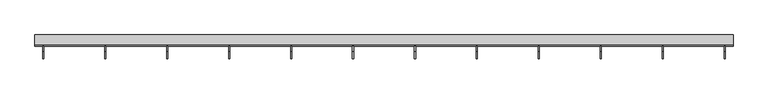
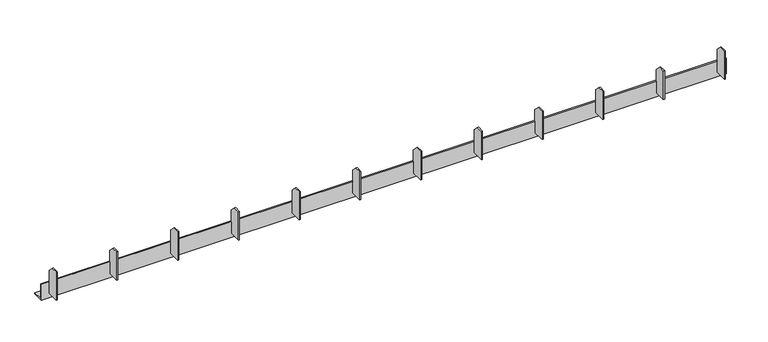
"""IFC4 building model written with IfcOpenShell, lengths in millimetres: beam geometry, NLRS_31_SF_LIB_latei geveldrager staal-AV-CWV-MMBS-SRP_gen_rsf : geveldrager_gen."""

import ifcopenshell
import ifcopenshell.guid

model = None  # the IFC model being written
_history = None  # IfcOwnerHistory: only IFC2X3 demands one
_inside = {}  # id of a spatial element -> (the spatial element, [elements in it])
_under = {}  # id of a project, library or spatial element -> (it, [spatial elements below it])
_declared = {}  # id of a project -> (the project, [libraries it declares])
_typed = {}  # id of a type object -> (the type object, [elements of that type])
_made_of = {}  # id of a material, layer set ... -> (it, [elements and type objects made of it])


def new_model(schema):
    """Start an empty IFC model of exactly this schema.

    Asked for "IFC4X3", IfcOpenShell would pick the latest addendum, in which some entities
    have other attributes; the version numbers below select the first issue.
    IFC2X3 requires an IfcOwnerHistory on every rooted entity: one is made here for all.
    """
    global model, _history
    if schema == "IFC4X3":
        model = ifcopenshell.file(schema_version=(4, 3, 0, 0))
    else:
        model = ifcopenshell.file(schema=schema)
    _inside.clear()
    _under.clear()
    _declared.clear()
    _typed.clear()
    _made_of.clear()
    _history = None
    if model.schema == "IFC2X3":
        org = make("IfcOrganization", Name="unknown")
        user = make(
            "IfcPersonAndOrganization",
            ThePerson=make("IfcPerson", FamilyName="unknown"),
            TheOrganization=org,
        )
        app = make(
            "IfcApplication",
            ApplicationDeveloper=org,
            Version="unknown",
            ApplicationFullName="unknown",
            ApplicationIdentifier="unknown",
        )
        _history = make(
            "IfcOwnerHistory",
            OwningUser=user,
            OwningApplication=app,
            ChangeAction="ADDED",
            CreationDate=0,
        )
    return model


def make(cls, **values):
    """One entity of the class cls with the attributes given. An attribute that is None is left unset."""
    return model.create_entity(
        cls, **{name: value for name, value in values.items() if value is not None}
    )


def rooted(cls, **values):
    """An entity with a GlobalId (a new one), such as an element, a storey or a relation."""
    return make(cls, GlobalId=ifcopenshell.guid.new(), OwnerHistory=_history, **values)


def si_unit(unit_type, name, prefix=None):
    """IfcSIUnit, for example si_unit("LENGTHUNIT", "METRE", prefix="MILLI")."""
    return make("IfcSIUnit", UnitType=unit_type, Prefix=prefix, Name=name)


def assignment(units):
    """IfcUnitAssignment: the units of a project."""
    return None if units is None else make("IfcUnitAssignment", Units=units)


def point(xyz):
    """IfcCartesianPoint."""
    return None if xyz is None else make("IfcCartesianPoint", Coordinates=xyz)


def direction(xyz):
    """IfcDirection."""
    return None if xyz is None else make("IfcDirection", DirectionRatios=xyz)


def frame(location, z_axis=None, x_axis=None):
    """IfcAxis2Placement3D, a coordinate frame: its origin and axes. An axis left out is left unset."""
    return make(
        "IfcAxis2Placement3D",
        Location=point(location),
        Axis=direction(z_axis),
        RefDirection=direction(x_axis),
    )


def origin():
    """The frame at (0, 0, 0) with its axes left unset."""
    return frame((0.0, 0.0, 0.0))


def place(relative_to, where):
    """IfcLocalPlacement: puts the frame where relative to a parent placement (None: the world)."""
    return make(
        "IfcLocalPlacement", PlacementRelTo=relative_to, RelativePlacement=where
    )


def context(
    kind, dimensions, precision=None, world=None, true_north=None, identifier=None
):
    """IfcGeometricRepresentationContext, for example the 3D "Model" context."""
    return make(
        "IfcGeometricRepresentationContext",
        ContextIdentifier=identifier,
        ContextType=kind,
        CoordinateSpaceDimension=dimensions,
        Precision=precision,
        WorldCoordinateSystem=world,
        TrueNorth=true_north,
    )


def project(units=None, contexts=None):
    """IfcProject with its units and contexts."""
    return rooted(
        "IfcProject",
        Name="project",
        RepresentationContexts=contexts,
        UnitsInContext=assignment(units),
    )


def spatial(cls, under=None, at=None, **own):
    """A site, building, storey or space (cls), placed at a placement, below another one or the project."""
    s = rooted(cls, ObjectPlacement=at, **own)
    if under is not None:
        _under.setdefault(under.id(), (under, []))[1].append(s)
    return s


def polyline(points):
    """IfcPolyline through the points."""
    return make("IfcPolyline", Points=[point(p) for p in points])


def outline(outer, holes=None, kind="AREA"):
    """IfcArbitraryClosedProfileDef: a profile drawn as a closed curve; with holes, ...WithVoids."""
    if holes is None:
        return make("IfcArbitraryClosedProfileDef", ProfileType=kind, OuterCurve=outer)
    return make(
        "IfcArbitraryProfileDefWithVoids",
        ProfileType=kind,
        OuterCurve=outer,
        InnerCurves=holes,
    )


def extrude(swept, where, along, depth):
    """IfcExtrudedAreaSolid: the profile swept, set in the frame where, extruded along a direction by depth."""
    return make(
        "IfcExtrudedAreaSolid",
        SweptArea=swept,
        Position=where,
        ExtrudedDirection=direction(along),
        Depth=depth,
    )


def shape(context_of_items, identifier, shape_type, items):
    """IfcShapeRepresentation: the items that make up one representation, for example the "Body"."""
    return make(
        "IfcShapeRepresentation",
        ContextOfItems=context_of_items,
        RepresentationIdentifier=identifier,
        RepresentationType=shape_type,
        Items=items,
    )


def source(mapping_origin, context_of_items, identifier, shape_type, items):
    """IfcRepresentationMap: a shape defined once, which mapped items show again and again."""
    return make(
        "IfcRepresentationMap",
        MappingOrigin=mapping_origin,
        MappedRepresentation=shape(context_of_items, identifier, shape_type, items),
    )


def transform(
    local_origin,
    x_axis=None,
    y_axis=None,
    z_axis=None,
    scale=None,
    scale2=None,
    scale3=None,
    uniform=True,
):
    """IfcCartesianTransformationOperator3D, or its non-uniform kind. x_axis, y_axis, z_axis: its Axis1, 2, 3."""
    if uniform:
        return make(
            "IfcCartesianTransformationOperator3D",
            Axis1=direction(x_axis),
            Axis2=direction(y_axis),
            LocalOrigin=point(local_origin),
            Scale=scale,
            Axis3=direction(z_axis),
        )
    return make(
        "IfcCartesianTransformationOperator3DnonUniform",
        Axis1=direction(x_axis),
        Axis2=direction(y_axis),
        LocalOrigin=point(local_origin),
        Scale=scale,
        Axis3=direction(z_axis),
        Scale2=scale2,
        Scale3=scale3,
    )


def mapped(mapping_source, mapping_target):
    """IfcMappedItem: shows the shape of a source again, moved by a transform."""
    return make(
        "IfcMappedItem", MappingSource=mapping_source, MappingTarget=mapping_target
    )


def made_of(thing, what):
    """Note that an element or type object is made of a material, layer set ...; save() writes the relation."""
    if what is not None:
        _made_of.setdefault(what.id(), (what, []))[1].append(thing)
    return thing


def element(
    cls,
    number,
    at=None,
    inside=None,
    cuts=None,
    type_object=None,
    material=None,
    context=None,
    identifier="Body",
    shape_type=None,
    held_by="IfcProductDefinitionShape",
    body=None,
    shapes=None,
    **own,
):
    """One element of the class cls, such as IfcWall. Its Tag is "e" and its number.

    at: its placement. inside: the storey or other place that contains it. cuts: it is an
    opening in that element (IfcRelVoidsElement). A single representation is given by context,
    identifier, shape_type and body (its items); several are given by shapes. held_by: the class
    of the entity that holds the representations. save() writes the other relations.
    """
    e = rooted(cls, Tag="e%d" % number, ObjectPlacement=at, **own)
    if body is not None:
        shapes = [shape(context, identifier, shape_type, body)]
    if shapes is not None:
        e.Representation = make(held_by, Representations=shapes)
    if inside is not None:
        _inside.setdefault(inside.id(), (inside, []))[1].append(e)
    if cuts is not None:
        rooted(
            "IfcRelVoidsElement", RelatingBuildingElement=cuts, RelatedOpeningElement=e
        )
    if type_object is not None:
        _typed.setdefault(type_object.id(), (type_object, []))[1].append(e)
    return made_of(e, material)


def aggregate(whole, parts):
    """IfcRelAggregates: a whole, such as a stair, and the parts it consists of."""
    return rooted("IfcRelAggregates", RelatingObject=whole, RelatedObjects=parts)


def save(model, path):
    """Write the relations noted so far, then the file.

    IfcRelAggregates (storeys below a building ...), IfcRelContainedInSpatialStructure (elements
    in a storey), IfcRelDefinesByType, IfcRelAssociatesMaterial and IfcRelDeclares: one each for
    every whole, place, type object, material and project.
    """
    for whole, parts in _under.values():
        aggregate(whole, parts)
    for where, things in _inside.values():
        rooted(
            "IfcRelContainedInSpatialStructure",
            RelatedElements=things,
            RelatingStructure=where,
        )
    for kind, things in _typed.values():
        rooted("IfcRelDefinesByType", RelatedObjects=things, RelatingType=kind)
    for what, things in _made_of.values():
        rooted("IfcRelAssociatesMaterial", RelatedObjects=things, RelatingMaterial=what)
    for by, libraries in _declared.values():
        rooted("IfcRelDeclares", RelatingContext=by, RelatedDefinitions=libraries)
    model.write(path)


def beam_0e76cdc8(model_context):
    return source(origin(), model_context, "Body", "SweptSolid", [
        extrude(outline(polyline([(-70.0, -35.0), (-180.0, -35.0), (-180.0, 235.0), (-120.0, 235.0), (-70.0, 185.0), (-70.0, -35.0)])), frame((2461.8181818, 0.0, 0.0), z_axis=(1.0, 0.0, 0.0), x_axis=(0.0, 1.0, 0.0)), (0.0, 0.0, 1.0), 10.0),
        extrude(outline(polyline([(-70.0, -35.0), (-180.0, -35.0), (-180.0, 235.0), (-120.0, 235.0), (-70.0, 185.0), (-70.0, -35.0)])), frame((1913.6363636, 0.0, 0.0), z_axis=(1.0, 0.0, 0.0), x_axis=(0.0, 1.0, 0.0)), (0.0, 0.0, 1.0), 10.0),
        extrude(outline(polyline([(-70.0, -35.0), (-180.0, -35.0), (-180.0, 235.0), (-120.0, 235.0), (-70.0, 185.0), (-70.0, -35.0)])), frame((1365.4545455, 0.0, 0.0), z_axis=(1.0, 0.0, 0.0), x_axis=(0.0, 1.0, 0.0)), (0.0, 0.0, 1.0), 10.0),
        extrude(outline(polyline([(-70.0, -35.0), (-180.0, -35.0), (-180.0, 235.0), (-120.0, 235.0), (-70.0, 185.0), (-70.0, -35.0)])), frame((817.2727273, 0.0, 0.0), z_axis=(1.0, 0.0, 0.0), x_axis=(0.0, 1.0, 0.0)), (0.0, 0.0, 1.0), 10.0),
        extrude(outline(polyline([(-70.0, -35.0), (-180.0, -35.0), (-180.0, 235.0), (-120.0, 235.0), (-70.0, 185.0), (-70.0, -35.0)])), frame((269.0909091, 0.0, 0.0), z_axis=(1.0, 0.0, 0.0), x_axis=(0.0, 1.0, 0.0)), (0.0, 0.0, 1.0), 10.0),
        extrude(outline(polyline([(-70.0, -35.0), (-180.0, -35.0), (-180.0, 235.0), (-120.0, 235.0), (-70.0, 185.0), (-70.0, -35.0)])), frame((-279.0909091, 0.0, 0.0), z_axis=(1.0, 0.0, 0.0), x_axis=(0.0, 1.0, 0.0)), (0.0, 0.0, 1.0), 10.0),
        extrude(outline(polyline([(-70.0, -35.0), (-180.0, -35.0), (-180.0, 235.0), (-120.0, 235.0), (-70.0, 185.0), (-70.0, -35.0)])), frame((-827.2727273, 0.0, 0.0), z_axis=(1.0, 0.0, 0.0), x_axis=(0.0, 1.0, 0.0)), (0.0, 0.0, 1.0), 10.0),
        extrude(outline(polyline([(-70.0, -35.0), (-180.0, -35.0), (-180.0, 235.0), (-120.0, 235.0), (-70.0, 185.0), (-70.0, -35.0)])), frame((-1375.4545455, 0.0, 0.0), z_axis=(1.0, 0.0, 0.0), x_axis=(0.0, 1.0, 0.0)), (0.0, 0.0, 1.0), 10.0),
        extrude(outline(polyline([(-70.0, -35.0), (-180.0, -35.0), (-180.0, 235.0), (-120.0, 235.0), (-70.0, 185.0), (-70.0, -35.0)])), frame((-1923.6363636, 0.0, 0.0), z_axis=(1.0, 0.0, 0.0), x_axis=(0.0, 1.0, 0.0)), (0.0, 0.0, 1.0), 10.0),
        extrude(outline(polyline([(-70.0, -35.0), (-180.0, -35.0), (-180.0, 235.0), (-120.0, 235.0), (-70.0, 185.0), (-70.0, -35.0)])), frame((-2471.8181818, 0.0, 0.0), z_axis=(1.0, 0.0, 0.0), x_axis=(0.0, 1.0, 0.0)), (0.0, 0.0, 1.0), 10.0),
        extrude(outline(polyline([(-70.0, -35.0), (-180.0, -35.0), (-180.0, 235.0), (-120.0, 235.0), (-70.0, 185.0), (-70.0, -35.0)])), frame((3010.0, 0.0, 0.0), z_axis=(1.0, 0.0, 0.0), x_axis=(0.0, 1.0, 0.0)), (0.0, 0.0, 1.0), 10.0),
        extrude(outline(polyline([(-70.0, -35.0), (-180.0, -35.0), (-180.0, 235.0), (-120.0, 235.0), (-70.0, 185.0), (-70.0, -35.0)])), frame((-3020.0, 0.0, 0.0), z_axis=(1.0, 0.0, 0.0), x_axis=(0.0, 1.0, 0.0)), (0.0, 0.0, 1.0), 10.0),
        extrude(outline(polyline([(-70.0, -75.0), (-70.0, 75.0), (-60.0, 75.0), (-60.0, -65.0), (30.0, -65.0), (30.0, -75.0), (-70.0, -75.0)])), frame((-3090.0, 0.0, 0.0), z_axis=(1.0, 0.0, 0.0), x_axis=(0.0, 1.0, 0.0)), (0.0, 0.0, 1.0), 6180.0),
    ])


if __name__ == "__main__":
    model = new_model("IFC4")
    model_context = context("Model", 3, world=origin())
    ifc_project = project(units=[si_unit("LENGTHUNIT", "METRE", prefix="MILLI")], contexts=[model_context])
    site = spatial("IfcSite", under=ifc_project)
    building = spatial("IfcBuilding", under=site)
    placement = place(None, origin())
    beam_shape = beam_0e76cdc8(model_context)
    element("IfcBeam", 1, ObjectType="NLRS_31_SF_LIB_latei geveldrager staal-AV-CWV-MMBS-SRP_gen_rsf : geveldrager_gen", at=placement, inside=building, context=model_context, shape_type="MappedRepresentation", body=[
        mapped(beam_shape, transform((0.0, 0.0, 0.0), x_axis=(1.0, 0.0, 0.0), y_axis=(0.0, 1.0, 0.0), z_axis=(0.0, 0.0, 1.0))),
    ])
    save(model, "model.ifc")

# Revit data of these elements
# Type "NLRS_31_SF_LIB_latei geveldrager staal-AV-CWV-MMBS-SRP_gen_rsf : geveldrager_gen"
#   Type IfcGUID = "19kvldyMP0rwUi5k27wrdj"
#   IfcExportAs = "IfcBeamType"
#   Type Comments = "geveldrager"
#   Model = "LOD200"
#   Description = "geveldrager vlgs leverancier"
#   Assembly Code = "31.10"
#   spouw_diepte [instance default] = 140 mm
#   hart_metselwerk [instance default] = 190 mm
#   r = 13 mm
#   console_hoogte [instance default] = 270 mm
#   console_eindafstand [instance default] = 75 mm
#   console_breedte [instance default] = 110 mm
#   console_beginafstand [instance default] = 75 mm
#   onderzijde_metselwerk_vanaf_vloer [instance default] = 300 mm
#   consoles_hoh [instance default] = 1000 mm
#   NLRS_C_lengte [instance default] = 1500 mm
#   Length [instance default] = 1500 mm
#   b = 100 mm
#   h = 150 mm
#   t = 10 mm
#   x = 70 mm
#   y = 75 mm
#   aantal [instance default] = 2
#   LOD300 = no
#   LOD200 = yes
#   Structural Material = NLRS_h2_staal_gen_rsf
# Element 1 (IfcBeam, "NLRS_31_SF_LIB_latei geveldrager staal-AV-CWV-MMBS-SRP_gen_rsf : geveldrager_gen")
#   consoles_hoh = 500 mm
#   NLRS_C_lengte = 6200 mm
#   aantal = 12
#   Materials on its faces: "NLRS_h2_staal_gen_rsf"
# Materials
#   "NLRS_h2_staal_gen_rsf": class "H - Metaal", colour RGB 189 187 185, transparency 0, Keynote = "h2", Manufacturer = "Revit Standards Foundation", URL = "www.revitstandards.org", Description = "staal", Cost = 0
